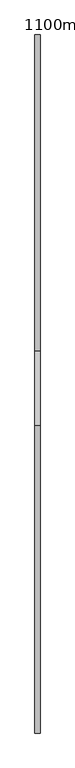
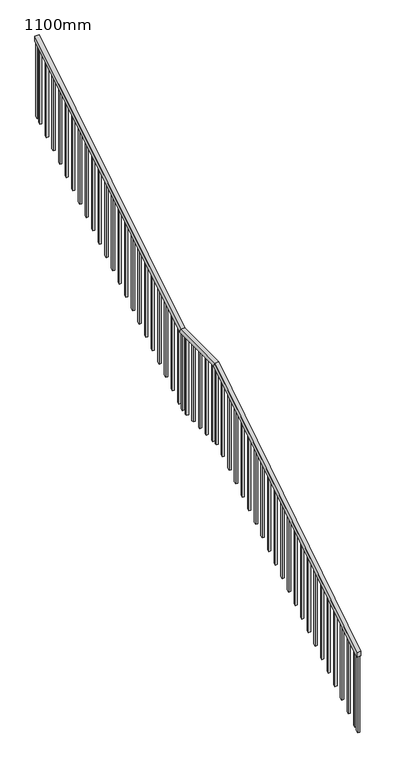
"""IFC4 building model written with IfcOpenShell, lengths in millimetres: railing geometry, 1100mm."""

from ifc_helpers import new_model, si_unit, frame, origin, place, context, project, spatial, polyline, outline, extrude, faceted_brep, source, transform, mapped, element, save


def railing_1100mm_2fb11b6b(model_context):
    return source(origin(), model_context, "Body", "SolidModel", [
        faceted_brep([(-22150.0159097, -6684.456375, 1268.797954), (-22150.0159097, -6684.456375, 1209.4512039), (-22100.0159097, -6684.456375, 1209.4512039), (-22100.0159097, -6684.456375, 1268.797954), (-22150.0159097, -3684.456375, 3186.9565217), (-22150.0159097, -3669.8380579, 3136.9565217), (-22100.0159097, -3669.8380579, 3136.9565217), (-22100.0159097, -3684.456375, 3186.9565217), (-22150.0159097, -2964.456375, 3186.9565217), (-22150.0159097, -2950.192194, 3136.9565217), (-22100.0159097, -2950.192194, 3136.9565217), (-22100.0159097, -2964.456375, 3186.9565217), (-22150.0159097, 115.543625, 5100.0), (-22100.0159097, 115.543625, 5100.0), (-22100.0159097, 115.543625, 5041.1402603), (-22150.0159097, 115.543625, 5041.1402603)], [[[0, 1, 2, 3]], [[1, 0, 4, 5]], [[2, 1, 5, 6]], [[3, 2, 6, 7]], [[0, 3, 7, 4]], [[5, 4, 8, 9]], [[6, 5, 9, 10]], [[7, 6, 10, 11]], [[4, 7, 11, 8]], [[12, 13, 14, 15]], [[9, 8, 12, 15]], [[10, 9, 15, 14]], [[11, 10, 14, 13]], [[8, 11, 13, 12]]]),
        extrude(outline(polyline([(33.043625, 4989.8980242), (58.043625, 5005.4259745), (58.043625, 4024.5530048), (33.043625, 4009.0250545), (33.043625, 4989.8980242)])), frame((-22137.5159097, 0.0, 0.0), z_axis=(1.0, 0.0, 0.0), x_axis=(0.0, 1.0, 0.0)), (0.0, 0.0, 1.0), 25.0),
        extrude(outline(polyline([(-106.956375, 4902.9415025), (-81.956375, 4918.4694528), (-81.956375, 3937.5964831), (-106.956375, 3922.0685328), (-106.956375, 4902.9415025)])), frame((-22137.5159097, 0.0, 0.0), z_axis=(1.0, 0.0, 0.0), x_axis=(0.0, 1.0, 0.0)), (0.0, 0.0, 1.0), 25.0),
        extrude(outline(polyline([(-246.956375, 4815.9849807), (-221.956375, 4831.5129311), (-221.956375, 3850.6399613), (-246.956375, 3835.112011), (-246.956375, 4815.9849807)])), frame((-22137.5159097, 0.0, 0.0), z_axis=(1.0, 0.0, 0.0), x_axis=(0.0, 1.0, 0.0)), (0.0, 0.0, 1.0), 25.0),
        extrude(outline(polyline([(-386.956375, 4729.028459), (-361.956375, 4744.5564093), (-361.956375, 3763.6834396), (-386.956375, 3748.1554893), (-386.956375, 4729.028459)])), frame((-22137.5159097, 0.0, 0.0), z_axis=(1.0, 0.0, 0.0), x_axis=(0.0, 1.0, 0.0)), (0.0, 0.0, 1.0), 25.0),
        extrude(outline(polyline([(-526.956375, 4642.0719373), (-501.956375, 4657.5998876), (-501.956375, 3676.7269179), (-526.956375, 3661.1989675), (-526.956375, 4642.0719373)])), frame((-22137.5159097, 0.0, 0.0), z_axis=(1.0, 0.0, 0.0), x_axis=(0.0, 1.0, 0.0)), (0.0, 0.0, 1.0), 25.0),
        extrude(outline(polyline([(-666.956375, 4555.1154155), (-641.956375, 4570.6433658), (-641.956375, 3589.7703961), (-666.956375, 3574.2424458), (-666.956375, 4555.1154155)])), frame((-22137.5159097, 0.0, 0.0), z_axis=(1.0, 0.0, 0.0), x_axis=(0.0, 1.0, 0.0)), (0.0, 0.0, 1.0), 25.0),
        extrude(outline(polyline([(-806.956375, 4468.1588938), (-781.956375, 4483.6868441), (-781.956375, 3502.8138744), (-806.956375, 3487.2859241), (-806.956375, 4468.1588938)])), frame((-22137.5159097, 0.0, 0.0), z_axis=(1.0, 0.0, 0.0), x_axis=(0.0, 1.0, 0.0)), (0.0, 0.0, 1.0), 25.0),
        extrude(outline(polyline([(-946.956375, 4381.2023721), (-921.956375, 4396.7303224), (-921.956375, 3415.8573526), (-946.956375, 3400.3294023), (-946.956375, 4381.2023721)])), frame((-22137.5159097, 0.0, 0.0), z_axis=(1.0, 0.0, 0.0), x_axis=(0.0, 1.0, 0.0)), (0.0, 0.0, 1.0), 25.0),
        extrude(outline(polyline([(-1086.956375, 4294.2458503), (-1061.956375, 4309.7738006), (-1061.956375, 3328.9008309), (-1086.956375, 3313.3728806), (-1086.956375, 4294.2458503)])), frame((-22137.5159097, 0.0, 0.0), z_axis=(1.0, 0.0, 0.0), x_axis=(0.0, 1.0, 0.0)), (0.0, 0.0, 1.0), 25.0),
        extrude(outline(polyline([(-1226.956375, 4207.2893286), (-1201.956375, 4222.8172789), (-1201.956375, 3241.9443092), (-1226.956375, 3226.4163588), (-1226.956375, 4207.2893286)])), frame((-22137.5159097, 0.0, 0.0), z_axis=(1.0, 0.0, 0.0), x_axis=(0.0, 1.0, 0.0)), (0.0, 0.0, 1.0), 25.0),
        extrude(outline(polyline([(-1366.956375, 4120.3328068), (-1341.956375, 4135.8607571), (-1341.956375, 3154.9877874), (-1366.956375, 3139.4598371), (-1366.956375, 4120.3328068)])), frame((-22137.5159097, 0.0, 0.0), z_axis=(1.0, 0.0, 0.0), x_axis=(0.0, 1.0, 0.0)), (0.0, 0.0, 1.0), 25.0),
        extrude(outline(polyline([(-1506.956375, 4033.3762851), (-1481.956375, 4048.9042354), (-1481.956375, 3068.0312657), (-1506.956375, 3052.5033154), (-1506.956375, 4033.3762851)])), frame((-22137.5159097, 0.0, 0.0), z_axis=(1.0, 0.0, 0.0), x_axis=(0.0, 1.0, 0.0)), (0.0, 0.0, 1.0), 25.0),
        extrude(outline(polyline([(-1646.956375, 3946.4197634), (-1621.956375, 3961.9477137), (-1621.956375, 2981.0747439), (-1646.956375, 2965.5467936), (-1646.956375, 3946.4197634)])), frame((-22137.5159097, 0.0, 0.0), z_axis=(1.0, 0.0, 0.0), x_axis=(0.0, 1.0, 0.0)), (0.0, 0.0, 1.0), 25.0),
        extrude(outline(polyline([(-1786.956375, 3859.4632416), (-1761.956375, 3874.9911919), (-1761.956375, 2894.1182222), (-1786.956375, 2878.5902719), (-1786.956375, 3859.4632416)])), frame((-22137.5159097, 0.0, 0.0), z_axis=(1.0, 0.0, 0.0), x_axis=(0.0, 1.0, 0.0)), (0.0, 0.0, 1.0), 25.0),
        extrude(outline(polyline([(-1926.956375, 3772.5067199), (-1901.956375, 3788.0346702), (-1901.956375, 2807.1617005), (-1926.956375, 2791.6337502), (-1926.956375, 3772.5067199)])), frame((-22137.5159097, 0.0, 0.0), z_axis=(1.0, 0.0, 0.0), x_axis=(0.0, 1.0, 0.0)), (0.0, 0.0, 1.0), 25.0),
        extrude(outline(polyline([(-2066.956375, 3685.5501981), (-2041.956375, 3701.0781484), (-2041.956375, 2720.2051787), (-2066.956375, 2704.6772284), (-2066.956375, 3685.5501981)])), frame((-22137.5159097, 0.0, 0.0), z_axis=(1.0, 0.0, 0.0), x_axis=(0.0, 1.0, 0.0)), (0.0, 0.0, 1.0), 25.0),
        extrude(outline(polyline([(-2206.956375, 3598.5936764), (-2181.956375, 3614.1216267), (-2181.956375, 2633.248657), (-2206.956375, 2617.7207067), (-2206.956375, 3598.5936764)])), frame((-22137.5159097, 0.0, 0.0), z_axis=(1.0, 0.0, 0.0), x_axis=(0.0, 1.0, 0.0)), (0.0, 0.0, 1.0), 25.0),
        extrude(outline(polyline([(-2346.956375, 3511.6371547), (-2321.956375, 3527.165105), (-2321.956375, 2546.2921352), (-2346.956375, 2530.7641849), (-2346.956375, 3511.6371547)])), frame((-22137.5159097, 0.0, 0.0), z_axis=(1.0, 0.0, 0.0), x_axis=(0.0, 1.0, 0.0)), (0.0, 0.0, 1.0), 25.0),
        extrude(outline(polyline([(-2486.956375, 3424.6806329), (-2461.956375, 3440.2085832), (-2461.956375, 2459.3356135), (-2486.956375, 2443.8076632), (-2486.956375, 3424.6806329)])), frame((-22137.5159097, 0.0, 0.0), z_axis=(1.0, 0.0, 0.0), x_axis=(0.0, 1.0, 0.0)), (0.0, 0.0, 1.0), 25.0),
        extrude(outline(polyline([(-2626.956375, 3337.7241112), (-2601.956375, 3353.2520615), (-2601.956375, 2372.3790918), (-2626.956375, 2356.8511415), (-2626.956375, 3337.7241112)])), frame((-22137.5159097, 0.0, 0.0), z_axis=(1.0, 0.0, 0.0), x_axis=(0.0, 1.0, 0.0)), (0.0, 0.0, 1.0), 25.0),
        extrude(outline(polyline([(-2766.956375, 3250.7675894), (-2741.956375, 3266.2955398), (-2741.956375, 2285.42257), (-2766.956375, 2269.8946197), (-2766.956375, 3250.7675894)])), frame((-22137.5159097, 0.0, 0.0), z_axis=(1.0, 0.0, 0.0), x_axis=(0.0, 1.0, 0.0)), (0.0, 0.0, 1.0), 25.0),
        extrude(outline(polyline([(-2906.956375, 3163.8110677), (-2881.956375, 3179.339018), (-2881.956375, 2198.4660483), (-2906.956375, 2182.938098), (-2906.956375, 3163.8110677)])), frame((-22137.5159097, 0.0, 0.0), z_axis=(1.0, 0.0, 0.0), x_axis=(0.0, 1.0, 0.0)), (0.0, 0.0, 1.0), 25.0),
        extrude(outline(polyline([(-22137.5159097, -3066.956375), (-22137.5159097, -3041.956375), (-22112.5159097, -3041.956375), (-22112.5159097, -3066.956375), (-22137.5159097, -3066.956375)])), frame((0.0, 0.0, 2133.5443962), z_axis=(0.0, 0.0, 1.0), x_axis=(1.0, 0.0, 0.0)), (0.0, 0.0, 1.0), 1003.4121256),
        extrude(outline(polyline([(-22137.5159097, -3206.956375), (-22137.5159097, -3181.956375), (-22112.5159097, -3181.956375), (-22112.5159097, -3206.956375), (-22137.5159097, -3206.956375)])), frame((0.0, 0.0, 2133.5443962), z_axis=(0.0, 0.0, 1.0), x_axis=(1.0, 0.0, 0.0)), (0.0, 0.0, 1.0), 1003.4121256),
        extrude(outline(polyline([(-22137.5159097, -3346.956375), (-22137.5159097, -3321.956375), (-22112.5159097, -3321.956375), (-22112.5159097, -3346.956375), (-22137.5159097, -3346.956375)])), frame((0.0, 0.0, 2133.5443962), z_axis=(0.0, 0.0, 1.0), x_axis=(1.0, 0.0, 0.0)), (0.0, 0.0, 1.0), 1003.4121256),
        extrude(outline(polyline([(-22137.5159097, -3486.956375), (-22137.5159097, -3461.956375), (-22112.5159097, -3461.956375), (-22112.5159097, -3486.956375), (-22137.5159097, -3486.956375)])), frame((0.0, 0.0, 2133.5443962), z_axis=(0.0, 0.0, 1.0), x_axis=(1.0, 0.0, 0.0)), (0.0, 0.0, 1.0), 1003.4121256),
        extrude(outline(polyline([(-22137.5159097, -3626.956375), (-22137.5159097, -3601.956375), (-22112.5159097, -3601.956375), (-22112.5159097, -3626.956375), (-22137.5159097, -3626.956375)])), frame((0.0, 0.0, 2133.5443962), z_axis=(0.0, 0.0, 1.0), x_axis=(1.0, 0.0, 0.0)), (0.0, 0.0, 1.0), 1003.4121256),
        extrude(outline(polyline([(-3826.956375, 3036.4972397), (-3801.956375, 3052.4818944), (-3801.956375, 2074.2831542), (-3826.956375, 2058.2984994), (-3826.956375, 3036.4972397)])), frame((-22137.5159097, 0.0, 0.0), z_axis=(1.0, 0.0, 0.0), x_axis=(0.0, 1.0, 0.0)), (0.0, 0.0, 1.0), 25.0),
        extrude(outline(polyline([(-3966.956375, 2946.9831732), (-3941.956375, 2962.9678279), (-3941.956375, 1984.7690877), (-3966.956375, 1968.7844329), (-3966.956375, 2946.9831732)])), frame((-22137.5159097, 0.0, 0.0), z_axis=(1.0, 0.0, 0.0), x_axis=(0.0, 1.0, 0.0)), (0.0, 0.0, 1.0), 25.0),
        extrude(outline(polyline([(-4106.956375, 2857.4691067), (-4081.956375, 2873.4537614), (-4081.956375, 1895.2550212), (-4106.956375, 1879.2703664), (-4106.956375, 2857.4691067)])), frame((-22137.5159097, 0.0, 0.0), z_axis=(1.0, 0.0, 0.0), x_axis=(0.0, 1.0, 0.0)), (0.0, 0.0, 1.0), 25.0),
        extrude(outline(polyline([(-4246.956375, 2767.9550402), (-4221.956375, 2783.9396949), (-4221.956375, 1805.7409547), (-4246.956375, 1789.7562999), (-4246.956375, 2767.9550402)])), frame((-22137.5159097, 0.0, 0.0), z_axis=(1.0, 0.0, 0.0), x_axis=(0.0, 1.0, 0.0)), (0.0, 0.0, 1.0), 25.0),
        extrude(outline(polyline([(-4386.956375, 2678.4409737), (-4361.956375, 2694.4256284), (-4361.956375, 1716.2268882), (-4386.956375, 1700.2422334), (-4386.956375, 2678.4409737)])), frame((-22137.5159097, 0.0, 0.0), z_axis=(1.0, 0.0, 0.0), x_axis=(0.0, 1.0, 0.0)), (0.0, 0.0, 1.0), 25.0),
        extrude(outline(polyline([(-4526.956375, 2588.9269072), (-4501.956375, 2604.9115619), (-4501.956375, 1626.7128217), (-4526.956375, 1610.7281669), (-4526.956375, 2588.9269072)])), frame((-22137.5159097, 0.0, 0.0), z_axis=(1.0, 0.0, 0.0), x_axis=(0.0, 1.0, 0.0)), (0.0, 0.0, 1.0), 25.0),
        extrude(outline(polyline([(-4666.956375, 2499.4128407), (-4641.956375, 2515.3974954), (-4641.956375, 1537.1987552), (-4666.956375, 1521.2141004), (-4666.956375, 2499.4128407)])), frame((-22137.5159097, 0.0, 0.0), z_axis=(1.0, 0.0, 0.0), x_axis=(0.0, 1.0, 0.0)), (0.0, 0.0, 1.0), 25.0),
        extrude(outline(polyline([(-4806.956375, 2409.8987742), (-4781.956375, 2425.8834289), (-4781.956375, 1447.6846887), (-4806.956375, 1431.700034), (-4806.956375, 2409.8987742)])), frame((-22137.5159097, 0.0, 0.0), z_axis=(1.0, 0.0, 0.0), x_axis=(0.0, 1.0, 0.0)), (0.0, 0.0, 1.0), 25.0),
        extrude(outline(polyline([(-4946.956375, 2320.3847077), (-4921.956375, 2336.3693624), (-4921.956375, 1358.1706222), (-4946.956375, 1342.1859675), (-4946.956375, 2320.3847077)])), frame((-22137.5159097, 0.0, 0.0), z_axis=(1.0, 0.0, 0.0), x_axis=(0.0, 1.0, 0.0)), (0.0, 0.0, 1.0), 25.0),
        extrude(outline(polyline([(-5086.956375, 2230.8706412), (-5061.956375, 2246.8552959), (-5061.956375, 1268.6565557), (-5086.956375, 1252.671901), (-5086.956375, 2230.8706412)])), frame((-22137.5159097, 0.0, 0.0), z_axis=(1.0, 0.0, 0.0), x_axis=(0.0, 1.0, 0.0)), (0.0, 0.0, 1.0), 25.0),
        extrude(outline(polyline([(-5226.956375, 2141.3565747), (-5201.956375, 2157.3412294), (-5201.956375, 1179.1424892), (-5226.956375, 1163.1578345), (-5226.956375, 2141.3565747)])), frame((-22137.5159097, 0.0, 0.0), z_axis=(1.0, 0.0, 0.0), x_axis=(0.0, 1.0, 0.0)), (0.0, 0.0, 1.0), 25.0),
        extrude(outline(polyline([(-5366.956375, 2051.8425082), (-5341.956375, 2067.8271629), (-5341.956375, 1089.6284227), (-5366.956375, 1073.643768), (-5366.956375, 2051.8425082)])), frame((-22137.5159097, 0.0, 0.0), z_axis=(1.0, 0.0, 0.0), x_axis=(0.0, 1.0, 0.0)), (0.0, 0.0, 1.0), 25.0),
        extrude(outline(polyline([(-5506.956375, 1962.3284417), (-5481.956375, 1978.3130964), (-5481.956375, 1000.1143562), (-5506.956375, 984.1297015), (-5506.956375, 1962.3284417)])), frame((-22137.5159097, 0.0, 0.0), z_axis=(1.0, 0.0, 0.0), x_axis=(0.0, 1.0, 0.0)), (0.0, 0.0, 1.0), 25.0),
        extrude(outline(polyline([(-5646.956375, 1872.8143752), (-5621.956375, 1888.79903), (-5621.956375, 910.6002897), (-5646.956375, 894.615635), (-5646.956375, 1872.8143752)])), frame((-22137.5159097, 0.0, 0.0), z_axis=(1.0, 0.0, 0.0), x_axis=(0.0, 1.0, 0.0)), (0.0, 0.0, 1.0), 25.0),
        extrude(outline(polyline([(-5786.956375, 1783.3003087), (-5761.956375, 1799.2849635), (-5761.956375, 821.0862232), (-5786.956375, 805.1015685), (-5786.956375, 1783.3003087)])), frame((-22137.5159097, 0.0, 0.0), z_axis=(1.0, 0.0, 0.0), x_axis=(0.0, 1.0, 0.0)), (0.0, 0.0, 1.0), 25.0),
        extrude(outline(polyline([(-5926.956375, 1693.7862422), (-5901.956375, 1709.770897), (-5901.956375, 731.5721567), (-5926.956375, 715.587502), (-5926.956375, 1693.7862422)])), frame((-22137.5159097, 0.0, 0.0), z_axis=(1.0, 0.0, 0.0), x_axis=(0.0, 1.0, 0.0)), (0.0, 0.0, 1.0), 25.0),
        extrude(outline(polyline([(-6066.956375, 1604.2721757), (-6041.956375, 1620.2568305), (-6041.956375, 642.0580902), (-6066.956375, 626.0734355), (-6066.956375, 1604.2721757)])), frame((-22137.5159097, 0.0, 0.0), z_axis=(1.0, 0.0, 0.0), x_axis=(0.0, 1.0, 0.0)), (0.0, 0.0, 1.0), 25.0),
        extrude(outline(polyline([(-6206.956375, 1514.7581092), (-6181.956375, 1530.742764), (-6181.956375, 552.5440237), (-6206.956375, 536.559369), (-6206.956375, 1514.7581092)])), frame((-22137.5159097, 0.0, 0.0), z_axis=(1.0, 0.0, 0.0), x_axis=(0.0, 1.0, 0.0)), (0.0, 0.0, 1.0), 25.0),
        extrude(outline(polyline([(-6346.956375, 1425.2440427), (-6321.956375, 1441.2286975), (-6321.956375, 463.0299572), (-6346.956375, 447.0453025), (-6346.956375, 1425.2440427)])), frame((-22137.5159097, 0.0, 0.0), z_axis=(1.0, 0.0, 0.0), x_axis=(0.0, 1.0, 0.0)), (0.0, 0.0, 1.0), 25.0),
        extrude(outline(polyline([(-6486.956375, 1335.7299762), (-6461.956375, 1351.714631), (-6461.956375, 373.5158907), (-6486.956375, 357.531236), (-6486.956375, 1335.7299762)])), frame((-22137.5159097, 0.0, 0.0), z_axis=(1.0, 0.0, 0.0), x_axis=(0.0, 1.0, 0.0)), (0.0, 0.0, 1.0), 25.0),
        extrude(outline(polyline([(-6626.956375, 1246.2159097), (-6601.956375, 1262.2005645), (-6601.956375, 284.0018242), (-6626.956375, 268.0171695), (-6626.956375, 1246.2159097)])), frame((-22137.5159097, 0.0, 0.0), z_axis=(1.0, 0.0, 0.0), x_axis=(0.0, 1.0, 0.0)), (0.0, 0.0, 1.0), 25.0),
        extrude(outline(polyline([(-2976.956375, 3136.9565217), (-2951.956375, 3136.9565217), (-2951.956375, 2154.9877874), (-2976.956375, 2139.4598371), (-2976.956375, 3136.9565217)])), frame((-22137.5159097, 0.0, 0.0), z_axis=(1.0, 0.0, 0.0), x_axis=(0.0, 1.0, 0.0)), (0.0, 0.0, 1.0), 25.0),
        extrude(outline(polyline([(-3696.956375, 3119.6174443), (-3671.956375, 3135.602099), (-3671.956375, 2133.5443962), (-3696.956375, 2133.5443962), (-3696.956375, 3119.6174443)])), frame((-22137.5159097, 0.0, 0.0), z_axis=(1.0, 0.0, 0.0), x_axis=(0.0, 1.0, 0.0)), (0.0, 0.0, 1.0), 25.0),
        extrude(outline(polyline([(90.543625, 5025.6123099), (115.543625, 5041.1402603), (115.543625, 4060.2672905), (90.543625, 4044.7393402), (90.543625, 5025.6123099)])), frame((-22137.5159097, 0.0, 0.0), z_axis=(1.0, 0.0, 0.0), x_axis=(0.0, 1.0, 0.0)), (0.0, 0.0, 1.0), 25.0),
        extrude(outline(polyline([(-6684.456375, 1209.4512039), (-6659.456375, 1225.4358586), (-6659.456375, 247.2371184), (-6684.456375, 231.2524636), (-6684.456375, 1209.4512039)])), frame((-22137.5159097, 0.0, 0.0), z_axis=(1.0, 0.0, 0.0), x_axis=(0.0, 1.0, 0.0)), (0.0, 0.0, 1.0), 25.0),
    ])


if __name__ == "__main__":
    model = new_model("IFC4")
    model_context = context("Model", 3, world=origin())
    ifc_project = project(units=[si_unit("LENGTHUNIT", "METRE", prefix="MILLI")], contexts=[model_context])
    site = spatial("IfcSite", under=ifc_project)
    building = spatial("IfcBuilding", under=site)
    placement = place(None, origin())
    railing_1100mm_shape = railing_1100mm_2fb11b6b(model_context)
    element("IfcRailing", 1, ObjectType="1100mm", at=placement, inside=building, context=model_context, shape_type="MappedRepresentation", body=[
        mapped(railing_1100mm_shape, transform((0.0, 0.0, 0.0), x_axis=(1.0, 0.0, 0.0), y_axis=(0.0, 1.0, 0.0), z_axis=(0.0, 0.0, 1.0))),
    ])
    save(model, "model.ifc")
